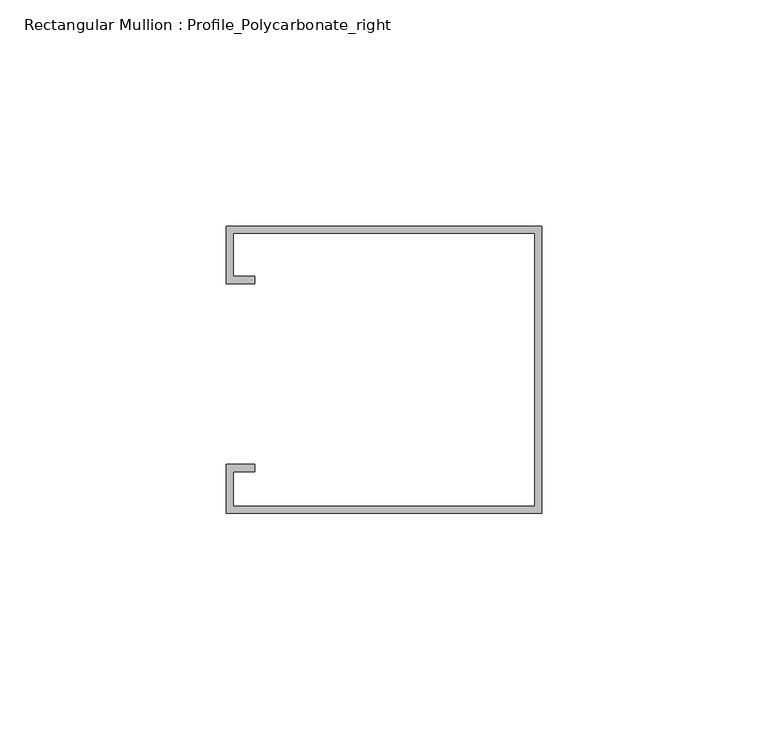
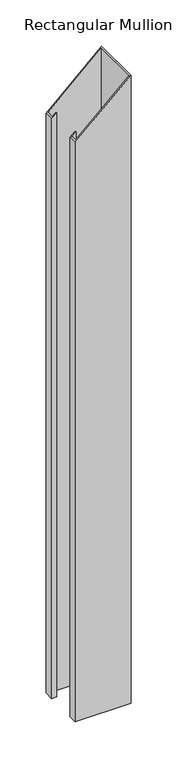
"""IFC4 building model written with IfcOpenShell, lengths in millimetres: member geometry, Rectangular Mullion : Profile_Polycarbonate_right."""

import ifcopenshell
import ifcopenshell.guid

model = None  # the IFC model being written
_history = None  # IfcOwnerHistory: only IFC2X3 demands one
_inside = {}  # id of a spatial element -> (the spatial element, [elements in it])
_under = {}  # id of a project, library or spatial element -> (it, [spatial elements below it])
_declared = {}  # id of a project -> (the project, [libraries it declares])
_typed = {}  # id of a type object -> (the type object, [elements of that type])
_made_of = {}  # id of a material, layer set ... -> (it, [elements and type objects made of it])


def new_model(schema):
    """Start an empty IFC model of exactly this schema.

    Asked for "IFC4X3", IfcOpenShell would pick the latest addendum, in which some entities
    have other attributes; the version numbers below select the first issue.
    IFC2X3 requires an IfcOwnerHistory on every rooted entity: one is made here for all.
    """
    global model, _history
    if schema == "IFC4X3":
        model = ifcopenshell.file(schema_version=(4, 3, 0, 0))
    else:
        model = ifcopenshell.file(schema=schema)
    _inside.clear()
    _under.clear()
    _declared.clear()
    _typed.clear()
    _made_of.clear()
    _history = None
    if model.schema == "IFC2X3":
        org = make("IfcOrganization", Name="unknown")
        user = make(
            "IfcPersonAndOrganization",
            ThePerson=make("IfcPerson", FamilyName="unknown"),
            TheOrganization=org,
        )
        app = make(
            "IfcApplication",
            ApplicationDeveloper=org,
            Version="unknown",
            ApplicationFullName="unknown",
            ApplicationIdentifier="unknown",
        )
        _history = make(
            "IfcOwnerHistory",
            OwningUser=user,
            OwningApplication=app,
            ChangeAction="ADDED",
            CreationDate=0,
        )
    return model


def make(cls, **values):
    """One entity of the class cls with the attributes given. An attribute that is None is left unset."""
    return model.create_entity(
        cls, **{name: value for name, value in values.items() if value is not None}
    )


def rooted(cls, **values):
    """An entity with a GlobalId (a new one), such as an element, a storey or a relation."""
    return make(cls, GlobalId=ifcopenshell.guid.new(), OwnerHistory=_history, **values)


def si_unit(unit_type, name, prefix=None):
    """IfcSIUnit, for example si_unit("LENGTHUNIT", "METRE", prefix="MILLI")."""
    return make("IfcSIUnit", UnitType=unit_type, Prefix=prefix, Name=name)


def assignment(units):
    """IfcUnitAssignment: the units of a project."""
    return None if units is None else make("IfcUnitAssignment", Units=units)


def point(xyz):
    """IfcCartesianPoint."""
    return None if xyz is None else make("IfcCartesianPoint", Coordinates=xyz)


def direction(xyz):
    """IfcDirection."""
    return None if xyz is None else make("IfcDirection", DirectionRatios=xyz)


def frame(location, z_axis=None, x_axis=None):
    """IfcAxis2Placement3D, a coordinate frame: its origin and axes. An axis left out is left unset."""
    return make(
        "IfcAxis2Placement3D",
        Location=point(location),
        Axis=direction(z_axis),
        RefDirection=direction(x_axis),
    )


def origin():
    """The frame at (0, 0, 0) with its axes left unset."""
    return frame((0.0, 0.0, 0.0))


def place(relative_to, where):
    """IfcLocalPlacement: puts the frame where relative to a parent placement (None: the world)."""
    return make(
        "IfcLocalPlacement", PlacementRelTo=relative_to, RelativePlacement=where
    )


def context(
    kind, dimensions, precision=None, world=None, true_north=None, identifier=None
):
    """IfcGeometricRepresentationContext, for example the 3D "Model" context."""
    return make(
        "IfcGeometricRepresentationContext",
        ContextIdentifier=identifier,
        ContextType=kind,
        CoordinateSpaceDimension=dimensions,
        Precision=precision,
        WorldCoordinateSystem=world,
        TrueNorth=true_north,
    )


def project(units=None, contexts=None):
    """IfcProject with its units and contexts."""
    return rooted(
        "IfcProject",
        Name="project",
        RepresentationContexts=contexts,
        UnitsInContext=assignment(units),
    )


def spatial(cls, under=None, at=None, **own):
    """A site, building, storey or space (cls), placed at a placement, below another one or the project."""
    s = rooted(cls, ObjectPlacement=at, **own)
    if under is not None:
        _under.setdefault(under.id(), (under, []))[1].append(s)
    return s


def faces_of(points, faces, orient=None, outer=None):
    """IfcFace entities. A face is a list of loops; a loop is a list of indices into points, from 0.

    orient and outer hold one flag for each loop. By default every Orientation is true, the
    first loop of a face is its IfcFaceOuterBound and the others are IfcFaceBound.
    """
    made = []
    for i, loops in enumerate(faces):
        bounds = []
        for j, loop in enumerate(loops):
            is_outer = j == 0 if outer is None else outer[i][j]
            bounds.append(
                make(
                    "IfcFaceOuterBound" if is_outer else "IfcFaceBound",
                    Bound=make("IfcPolyLoop", Polygon=[points[k] for k in loop]),
                    Orientation=True if orient is None else orient[i][j],
                )
            )
        made.append(make("IfcFace", Bounds=bounds))
    return made


def faceted_brep(points, faces, orient=None, outer=None, voids=None):
    """IfcFacetedBrep: a solid bounded by flat faces; with voids (closed shells), ...WithVoids."""
    shared = [point(p) for p in points]
    hull = make("IfcClosedShell", CfsFaces=faces_of(shared, faces, orient, outer))
    if voids is None:
        return make("IfcFacetedBrep", Outer=hull)
    return make(
        "IfcFacetedBrepWithVoids",
        Outer=hull,
        Voids=[
            make(cls, CfsFaces=faces_of(shared, fs, o, b)) for cls, fs, o, b in voids
        ],
    )


def shape(context_of_items, identifier, shape_type, items):
    """IfcShapeRepresentation: the items that make up one representation, for example the "Body"."""
    return make(
        "IfcShapeRepresentation",
        ContextOfItems=context_of_items,
        RepresentationIdentifier=identifier,
        RepresentationType=shape_type,
        Items=items,
    )


def source(mapping_origin, context_of_items, identifier, shape_type, items):
    """IfcRepresentationMap: a shape defined once, which mapped items show again and again."""
    return make(
        "IfcRepresentationMap",
        MappingOrigin=mapping_origin,
        MappedRepresentation=shape(context_of_items, identifier, shape_type, items),
    )


def transform(
    local_origin,
    x_axis=None,
    y_axis=None,
    z_axis=None,
    scale=None,
    scale2=None,
    scale3=None,
    uniform=True,
):
    """IfcCartesianTransformationOperator3D, or its non-uniform kind. x_axis, y_axis, z_axis: its Axis1, 2, 3."""
    if uniform:
        return make(
            "IfcCartesianTransformationOperator3D",
            Axis1=direction(x_axis),
            Axis2=direction(y_axis),
            LocalOrigin=point(local_origin),
            Scale=scale,
            Axis3=direction(z_axis),
        )
    return make(
        "IfcCartesianTransformationOperator3DnonUniform",
        Axis1=direction(x_axis),
        Axis2=direction(y_axis),
        LocalOrigin=point(local_origin),
        Scale=scale,
        Axis3=direction(z_axis),
        Scale2=scale2,
        Scale3=scale3,
    )


def mapped(mapping_source, mapping_target):
    """IfcMappedItem: shows the shape of a source again, moved by a transform."""
    return make(
        "IfcMappedItem", MappingSource=mapping_source, MappingTarget=mapping_target
    )


def made_of(thing, what):
    """Note that an element or type object is made of a material, layer set ...; save() writes the relation."""
    if what is not None:
        _made_of.setdefault(what.id(), (what, []))[1].append(thing)
    return thing


def element(
    cls,
    number,
    at=None,
    inside=None,
    cuts=None,
    type_object=None,
    material=None,
    context=None,
    identifier="Body",
    shape_type=None,
    held_by="IfcProductDefinitionShape",
    body=None,
    shapes=None,
    **own,
):
    """One element of the class cls, such as IfcWall. Its Tag is "e" and its number.

    at: its placement. inside: the storey or other place that contains it. cuts: it is an
    opening in that element (IfcRelVoidsElement). A single representation is given by context,
    identifier, shape_type and body (its items); several are given by shapes. held_by: the class
    of the entity that holds the representations. save() writes the other relations.
    """
    e = rooted(cls, Tag="e%d" % number, ObjectPlacement=at, **own)
    if body is not None:
        shapes = [shape(context, identifier, shape_type, body)]
    if shapes is not None:
        e.Representation = make(held_by, Representations=shapes)
    if inside is not None:
        _inside.setdefault(inside.id(), (inside, []))[1].append(e)
    if cuts is not None:
        rooted(
            "IfcRelVoidsElement", RelatingBuildingElement=cuts, RelatedOpeningElement=e
        )
    if type_object is not None:
        _typed.setdefault(type_object.id(), (type_object, []))[1].append(e)
    return made_of(e, material)


def aggregate(whole, parts):
    """IfcRelAggregates: a whole, such as a stair, and the parts it consists of."""
    return rooted("IfcRelAggregates", RelatingObject=whole, RelatedObjects=parts)


def save(model, path):
    """Write the relations noted so far, then the file.

    IfcRelAggregates (storeys below a building ...), IfcRelContainedInSpatialStructure (elements
    in a storey), IfcRelDefinesByType, IfcRelAssociatesMaterial and IfcRelDeclares: one each for
    every whole, place, type object, material and project.
    """
    for whole, parts in _under.values():
        aggregate(whole, parts)
    for where, things in _inside.values():
        rooted(
            "IfcRelContainedInSpatialStructure",
            RelatedElements=things,
            RelatingStructure=where,
        )
    for kind, things in _typed.values():
        rooted("IfcRelDefinesByType", RelatedObjects=things, RelatingType=kind)
    for what, things in _made_of.values():
        rooted("IfcRelAssociatesMaterial", RelatedObjects=things, RelatingMaterial=what)
    for by, libraries in _declared.values():
        rooted("IfcRelDeclares", RelatingContext=by, RelatedDefinitions=libraries)
    model.write(path)


def rectangular_mullion_profile_polycarbonate_right_7a9c6186(model_context):
    return source(origin(), model_context, "Body", "Brep", [
        faceted_brep([(0.0, 32.7, -832.3791667), (0.0, -30.8, -832.3791667), (-69.85, -30.8, -832.3791667), (-69.85, -20.0, -832.3791667), (-63.5, -20.0, -832.3791667), (-63.5, -21.5875, -832.3791667), (-68.2625, -21.5875, -832.3791667), (-68.2625, -29.2125, -832.3791667), (-1.5875, -29.2125, -832.3791667), (-1.5875, 31.1125, -832.3791667), (-68.2625, 31.1125, -832.3791667), (-68.2625, 21.5875, -832.3791667), (-63.5, 21.5875, -832.3791667), (-63.5, 20.0, -832.3791667), (-69.85, 20.0, -832.3791667), (-69.85, 32.7, -832.3791667), (-69.85, 32.7, -64.2712818), (0.0, 32.7, 0.0), (-69.85, 20.0, -64.2712818), (-63.5, 20.0, -58.428438), (-63.5, 21.5875, -58.428438), (-68.2625, 21.5875, -62.8105708), (-68.2625, 31.1125, -62.8105708), (-1.5875, 31.1125, -1.4607109), (-1.5875, -29.2125, -1.4607109), (-68.2625, -29.2125, -62.8105708), (-68.2625, -21.5875, -62.8105708), (-63.5, -21.5875, -58.428438), (-63.5, -20.0, -58.428438), (-69.85, -20.0, -64.2712818), (-69.85, -30.8, -64.2712818), (0.0, -30.8, 0.0)], [[[0, 1, 2, 3, 4, 5, 6, 7, 8, 9, 10, 11, 12, 13, 14, 15]], [[16, 17, 0, 15]], [[18, 16, 15, 14]], [[19, 18, 14, 13]], [[20, 19, 13, 12]], [[21, 20, 12, 11]], [[22, 21, 11, 10]], [[23, 22, 10, 9]], [[24, 23, 9, 8]], [[25, 24, 8, 7]], [[26, 25, 7, 6]], [[27, 26, 6, 5]], [[28, 27, 5, 4]], [[29, 28, 4, 3]], [[30, 29, 3, 2]], [[31, 30, 2, 1]], [[17, 31, 1, 0]], [[17, 16, 18, 19, 20, 21, 22, 23, 24, 25, 26, 27, 28, 29, 30, 31]]]),
    ])


if __name__ == "__main__":
    model = new_model("IFC4")
    model_context = context("Model", 3, world=origin())
    ifc_project = project(units=[si_unit("LENGTHUNIT", "METRE", prefix="MILLI")], contexts=[model_context])
    site = spatial("IfcSite", under=ifc_project)
    building = spatial("IfcBuilding", under=site)
    placement = place(None, origin())
    rectangular_mullion_profile_polycarbonate_right_shape = rectangular_mullion_profile_polycarbonate_right_7a9c6186(model_context)
    element("IfcMember", 1, ObjectType="Rectangular Mullion : Profile_Polycarbonate_right", at=placement, inside=building, context=model_context, shape_type="MappedRepresentation", body=[
        mapped(rectangular_mullion_profile_polycarbonate_right_shape, transform((0.0, 0.0, 0.0), x_axis=(1.0, 0.0, 0.0), y_axis=(0.0, 1.0, 0.0), z_axis=(0.0, 0.0, 1.0))),
    ])
    save(model, "model.ifc")

# Revit data of these elements
# Type "Rectangular Mullion : Profile_Polycarbonate_right"
#   built-in parameter 1007322 = 0.208333 (stored number, unit not read)
#   built-in parameter 1007321 = 0 (stored number, unit not read)
#   built-in parameter 1007320 = 0.00520833 (stored number, unit not read)
# Element 1 (IfcMember, "Rectangular Mullion : Profile_Polycarbonate_right")
#   Materials on its faces: "ALUMINUM PROFILE AT POLYCARBONATE PANEL"
# Materials
#   "ALUMINUM PROFILE AT POLYCARBONATE PANEL": class "Metal", colour RGB 244 244 244, transparency 0, Description = "Aluminum 6061", Cost = 0
